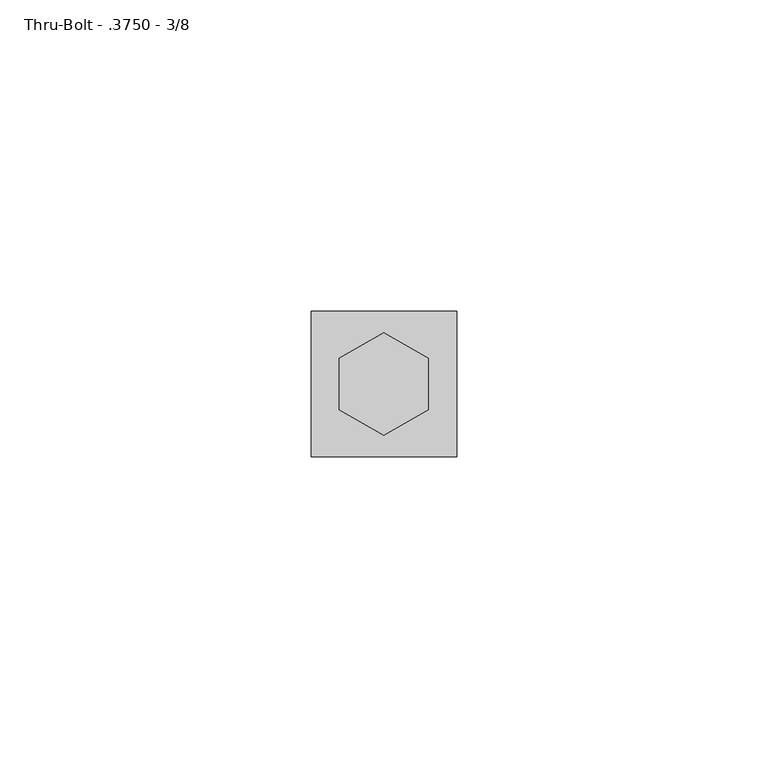
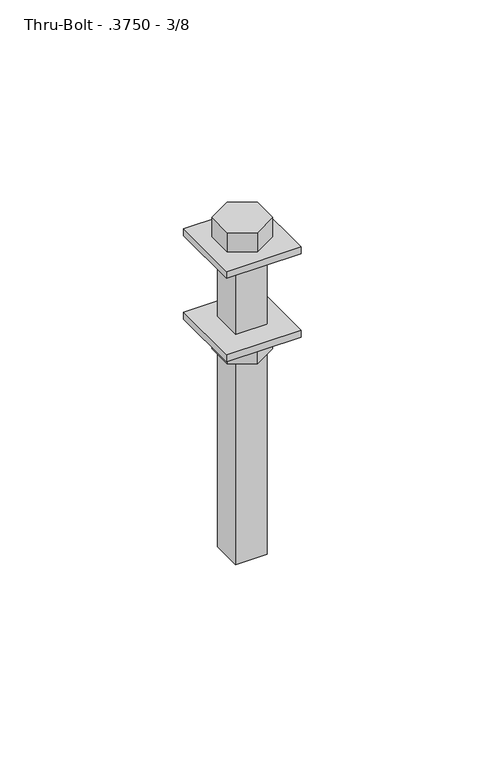
"""IFC4 building model written with IfcOpenShell, lengths in millimetres: fastener geometry, 060523 - W_P_C - Fastenings - Generic - SQUARE : Thru-Bolt - .3750 - 3/8."""

from ifc_helpers import new_model, si_unit, frame, origin, origin_with_axes, place, context, project, spatial, polyline, outline, extrude, source, transform, mapped, element, save


def thru_bolt_3750_3_8_48b59bf8(model_context):
    return source(origin(), model_context, "Body", "SweptSolid", [
        extrude(outline(polyline([(-11.7185281, -11.7185281), (-11.7185281, 11.7185281), (11.7185281, 11.7185281), (11.7185281, -11.7185281), (-11.7185281, -11.7185281)])), origin_with_axes(), (0.0, 0.0, 1.0), 2.2690667),
        extrude(outline(polyline([(-11.7185281, -11.7185281), (-11.7185281, 11.7185281), (11.7185281, 11.7185281), (11.7185281, -11.7185281), (-11.7185281, -11.7185281)])), frame((0.0, 0.0, -27.6690667), z_axis=(0.0, 0.0, 1.0), x_axis=(1.0, 0.0, 0.0)), (0.0, 0.0, 1.0), 2.2690667),
        extrude(outline(polyline([(-7.14375, -4.124446), (-7.14375, 4.124446), (0.0, 8.248892), (7.14375, 4.124446), (7.14375, -4.124446), (0.0, -8.248892), (-7.14375, -4.124446)])), frame((0.0, 0.0, -34.4762667), z_axis=(0.0, 0.0, 1.0), x_axis=(1.0, 0.0, 0.0)), (0.0, 0.0, 1.0), 6.8072),
        extrude(outline(polyline([(-7.14375, 4.124446), (0.0, 8.248892), (7.14375, 4.124446), (7.14375, -4.124446), (0.0, -8.248892), (-7.14375, -4.124446), (-7.14375, 4.124446)])), frame((0.0, 0.0, 2.2690667), z_axis=(0.0, 0.0, 1.0), x_axis=(1.0, 0.0, 0.0)), (0.0, 0.0, 1.0), 6.8072),
        extrude(outline(polyline([(-4.9113281, 4.9113281), (4.9113281, 4.9113281), (4.9113281, -4.9113281), (-4.9113281, -4.9113281), (-4.9113281, 4.9113281)])), frame((0.0, 0.0, -101.6), z_axis=(0.0, 0.0, 1.0), x_axis=(1.0, 0.0, 0.0)), (0.0, 0.0, 1.0), 103.8690667),
    ])


if __name__ == "__main__":
    model = new_model("IFC4")
    model_context = context("Model", 3, world=origin())
    ifc_project = project(units=[si_unit("LENGTHUNIT", "METRE", prefix="MILLI")], contexts=[model_context])
    site = spatial("IfcSite", under=ifc_project)
    building = spatial("IfcBuilding", under=site)
    placement = place(None, origin())
    thru_bolt_3750_3_8_shape = thru_bolt_3750_3_8_48b59bf8(model_context)
    element("IfcFastener", 1, ObjectType="060523 - W_P_C - Fastenings - Generic - SQUARE : Thru-Bolt - .3750 - 3/8", at=placement, inside=building, context=model_context, shape_type="MappedRepresentation", body=[
        mapped(thru_bolt_3750_3_8_shape, transform((0.0, 0.0, 0.0), x_axis=(1.0, 0.0, 0.0), y_axis=(0.0, 1.0, 0.0), z_axis=(0.0, 0.0, 1.0))),
    ])
    save(model, "model.ifc")

# Revit data of these elements
# Type "060523 - W_P_C - Fastenings - Generic - SQUARE : Thru-Bolt - .3750 - 3/8"
#   Washer_Thickness = 0' - 0.08933"
#   Washer Radius = 0' - 0.46136"
#   Washer Offset - Head = 0' - 0.08933"
#   Washer Offset = 0' - 0.08933"
#   Thickness_of_Substrate [instance default] = 0' - 1"
#   Side = 0' - 0.3252"
#   Radius = 0' - 0.19336"
#   Length [instance default] = 0' - 4"
#   Head Size = 0' - 0 9/16"
#   Head Radius = 0' - 0 9/32"
#   Head Height = 0' - 0.268"
#   Double Diameter = 0' - 0 99/128"
#   Diameter = 0' - 0 99/256"
#   Default Elevation = 4' - 0"
#   Washer_Nut_Visibility = yes
#   Washer_Head_Visibility = yes
#   Round_Head_Visibility = no
#   Point Visibility = no
#   Nut_Visibility = yes
#   Hex_Head_Visiblilty = yes
#   Washer Material = none
#   Bolt Material (Size) = AT SILL - FASTENER AT 24" O.C.
# Element 1 (IfcFastener, "060523 - W_P_C - Fastenings - Generic - SQUARE : Thru-Bolt - .3750 - 3/8")
#   Materials on its faces: "AT SILL - FASTENER AT 24\" O.C."
# Materials
#   "AT SILL - FASTENER AT 24\" O.C.": class "Generic", colour RGB 120 120 120, transparency 0, Cost = 0
